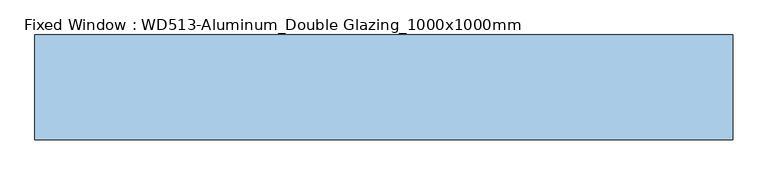
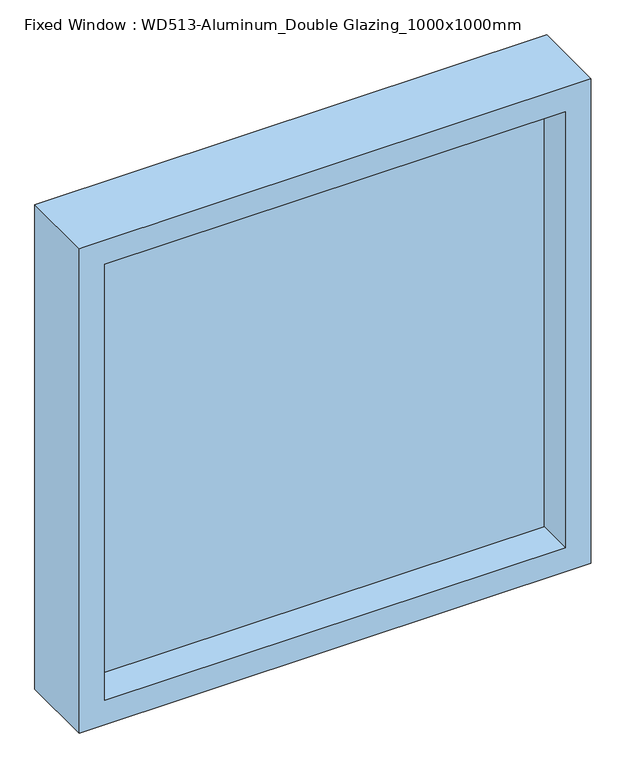
"""IFC4 building model written with IfcOpenShell, lengths in millimetres: window geometry, Fixed Window : WD513-Aluminum_Double Glazing_1000x1000mm."""

import ifcopenshell
import ifcopenshell.guid

model = None  # the IFC model being written
_history = None  # IfcOwnerHistory: only IFC2X3 demands one
_inside = {}  # id of a spatial element -> (the spatial element, [elements in it])
_under = {}  # id of a project, library or spatial element -> (it, [spatial elements below it])
_declared = {}  # id of a project -> (the project, [libraries it declares])
_typed = {}  # id of a type object -> (the type object, [elements of that type])
_made_of = {}  # id of a material, layer set ... -> (it, [elements and type objects made of it])


def new_model(schema):
    """Start an empty IFC model of exactly this schema.

    Asked for "IFC4X3", IfcOpenShell would pick the latest addendum, in which some entities
    have other attributes; the version numbers below select the first issue.
    IFC2X3 requires an IfcOwnerHistory on every rooted entity: one is made here for all.
    """
    global model, _history
    if schema == "IFC4X3":
        model = ifcopenshell.file(schema_version=(4, 3, 0, 0))
    else:
        model = ifcopenshell.file(schema=schema)
    _inside.clear()
    _under.clear()
    _declared.clear()
    _typed.clear()
    _made_of.clear()
    _history = None
    if model.schema == "IFC2X3":
        org = make("IfcOrganization", Name="unknown")
        user = make(
            "IfcPersonAndOrganization",
            ThePerson=make("IfcPerson", FamilyName="unknown"),
            TheOrganization=org,
        )
        app = make(
            "IfcApplication",
            ApplicationDeveloper=org,
            Version="unknown",
            ApplicationFullName="unknown",
            ApplicationIdentifier="unknown",
        )
        _history = make(
            "IfcOwnerHistory",
            OwningUser=user,
            OwningApplication=app,
            ChangeAction="ADDED",
            CreationDate=0,
        )
    return model


def make(cls, **values):
    """One entity of the class cls with the attributes given. An attribute that is None is left unset."""
    return model.create_entity(
        cls, **{name: value for name, value in values.items() if value is not None}
    )


def rooted(cls, **values):
    """An entity with a GlobalId (a new one), such as an element, a storey or a relation."""
    return make(cls, GlobalId=ifcopenshell.guid.new(), OwnerHistory=_history, **values)


def si_unit(unit_type, name, prefix=None):
    """IfcSIUnit, for example si_unit("LENGTHUNIT", "METRE", prefix="MILLI")."""
    return make("IfcSIUnit", UnitType=unit_type, Prefix=prefix, Name=name)


def assignment(units):
    """IfcUnitAssignment: the units of a project."""
    return None if units is None else make("IfcUnitAssignment", Units=units)


def point(xyz):
    """IfcCartesianPoint."""
    return None if xyz is None else make("IfcCartesianPoint", Coordinates=xyz)


def direction(xyz):
    """IfcDirection."""
    return None if xyz is None else make("IfcDirection", DirectionRatios=xyz)


def frame(location, z_axis=None, x_axis=None):
    """IfcAxis2Placement3D, a coordinate frame: its origin and axes. An axis left out is left unset."""
    return make(
        "IfcAxis2Placement3D",
        Location=point(location),
        Axis=direction(z_axis),
        RefDirection=direction(x_axis),
    )


def origin():
    """The frame at (0, 0, 0) with its axes left unset."""
    return frame((0.0, 0.0, 0.0))


def place(relative_to, where):
    """IfcLocalPlacement: puts the frame where relative to a parent placement (None: the world)."""
    return make(
        "IfcLocalPlacement", PlacementRelTo=relative_to, RelativePlacement=where
    )


def context(
    kind, dimensions, precision=None, world=None, true_north=None, identifier=None
):
    """IfcGeometricRepresentationContext, for example the 3D "Model" context."""
    return make(
        "IfcGeometricRepresentationContext",
        ContextIdentifier=identifier,
        ContextType=kind,
        CoordinateSpaceDimension=dimensions,
        Precision=precision,
        WorldCoordinateSystem=world,
        TrueNorth=true_north,
    )


def project(units=None, contexts=None):
    """IfcProject with its units and contexts."""
    return rooted(
        "IfcProject",
        Name="project",
        RepresentationContexts=contexts,
        UnitsInContext=assignment(units),
    )


def spatial(cls, under=None, at=None, **own):
    """A site, building, storey or space (cls), placed at a placement, below another one or the project."""
    s = rooted(cls, ObjectPlacement=at, **own)
    if under is not None:
        _under.setdefault(under.id(), (under, []))[1].append(s)
    return s


def polyline(points):
    """IfcPolyline through the points."""
    return make("IfcPolyline", Points=[point(p) for p in points])


def outline(outer, holes=None, kind="AREA"):
    """IfcArbitraryClosedProfileDef: a profile drawn as a closed curve; with holes, ...WithVoids."""
    if holes is None:
        return make("IfcArbitraryClosedProfileDef", ProfileType=kind, OuterCurve=outer)
    return make(
        "IfcArbitraryProfileDefWithVoids",
        ProfileType=kind,
        OuterCurve=outer,
        InnerCurves=holes,
    )


def extrude(swept, where, along, depth):
    """IfcExtrudedAreaSolid: the profile swept, set in the frame where, extruded along a direction by depth."""
    return make(
        "IfcExtrudedAreaSolid",
        SweptArea=swept,
        Position=where,
        ExtrudedDirection=direction(along),
        Depth=depth,
    )


def shape(context_of_items, identifier, shape_type, items):
    """IfcShapeRepresentation: the items that make up one representation, for example the "Body"."""
    return make(
        "IfcShapeRepresentation",
        ContextOfItems=context_of_items,
        RepresentationIdentifier=identifier,
        RepresentationType=shape_type,
        Items=items,
    )


def source(mapping_origin, context_of_items, identifier, shape_type, items):
    """IfcRepresentationMap: a shape defined once, which mapped items show again and again."""
    return make(
        "IfcRepresentationMap",
        MappingOrigin=mapping_origin,
        MappedRepresentation=shape(context_of_items, identifier, shape_type, items),
    )


def transform(
    local_origin,
    x_axis=None,
    y_axis=None,
    z_axis=None,
    scale=None,
    scale2=None,
    scale3=None,
    uniform=True,
):
    """IfcCartesianTransformationOperator3D, or its non-uniform kind. x_axis, y_axis, z_axis: its Axis1, 2, 3."""
    if uniform:
        return make(
            "IfcCartesianTransformationOperator3D",
            Axis1=direction(x_axis),
            Axis2=direction(y_axis),
            LocalOrigin=point(local_origin),
            Scale=scale,
            Axis3=direction(z_axis),
        )
    return make(
        "IfcCartesianTransformationOperator3DnonUniform",
        Axis1=direction(x_axis),
        Axis2=direction(y_axis),
        LocalOrigin=point(local_origin),
        Scale=scale,
        Axis3=direction(z_axis),
        Scale2=scale2,
        Scale3=scale3,
    )


def mapped(mapping_source, mapping_target):
    """IfcMappedItem: shows the shape of a source again, moved by a transform."""
    return make(
        "IfcMappedItem", MappingSource=mapping_source, MappingTarget=mapping_target
    )


def made_of(thing, what):
    """Note that an element or type object is made of a material, layer set ...; save() writes the relation."""
    if what is not None:
        _made_of.setdefault(what.id(), (what, []))[1].append(thing)
    return thing


def element(
    cls,
    number,
    at=None,
    inside=None,
    cuts=None,
    type_object=None,
    material=None,
    context=None,
    identifier="Body",
    shape_type=None,
    held_by="IfcProductDefinitionShape",
    body=None,
    shapes=None,
    **own,
):
    """One element of the class cls, such as IfcWall. Its Tag is "e" and its number.

    at: its placement. inside: the storey or other place that contains it. cuts: it is an
    opening in that element (IfcRelVoidsElement). A single representation is given by context,
    identifier, shape_type and body (its items); several are given by shapes. held_by: the class
    of the entity that holds the representations. save() writes the other relations.
    """
    e = rooted(cls, Tag="e%d" % number, ObjectPlacement=at, **own)
    if body is not None:
        shapes = [shape(context, identifier, shape_type, body)]
    if shapes is not None:
        e.Representation = make(held_by, Representations=shapes)
    if inside is not None:
        _inside.setdefault(inside.id(), (inside, []))[1].append(e)
    if cuts is not None:
        rooted(
            "IfcRelVoidsElement", RelatingBuildingElement=cuts, RelatedOpeningElement=e
        )
    if type_object is not None:
        _typed.setdefault(type_object.id(), (type_object, []))[1].append(e)
    return made_of(e, material)


def aggregate(whole, parts):
    """IfcRelAggregates: a whole, such as a stair, and the parts it consists of."""
    return rooted("IfcRelAggregates", RelatingObject=whole, RelatedObjects=parts)


def save(model, path):
    """Write the relations noted so far, then the file.

    IfcRelAggregates (storeys below a building ...), IfcRelContainedInSpatialStructure (elements
    in a storey), IfcRelDefinesByType, IfcRelAssociatesMaterial and IfcRelDeclares: one each for
    every whole, place, type object, material and project.
    """
    for whole, parts in _under.values():
        aggregate(whole, parts)
    for where, things in _inside.values():
        rooted(
            "IfcRelContainedInSpatialStructure",
            RelatedElements=things,
            RelatingStructure=where,
        )
    for kind, things in _typed.values():
        rooted("IfcRelDefinesByType", RelatedObjects=things, RelatingType=kind)
    for what, things in _made_of.values():
        rooted("IfcRelAssociatesMaterial", RelatedObjects=things, RelatingMaterial=what)
    for by, libraries in _declared.values():
        rooted("IfcRelDeclares", RelatingContext=by, RelatedDefinitions=libraries)
    model.write(path)


def fixed_window_wd513_aluminum_double_glazing_1000x1000mm_e073f05b(model_context):
    return source(origin(), model_context, "Body", "SweptSolid", [
        extrude(outline(polyline([(-450.0, 3.0), (450.0, 3.0), (450.0, -3.0), (-450.0, -3.0), (-450.0, 3.0)])), frame((0.0, 0.0, 850.0), z_axis=(0.0, 0.0, 1.0), x_axis=(1.0, 0.0, 0.0)), (0.0, 0.0, 1.0), 900.0),
        extrude(outline(polyline([(1800.0, -500.0), (800.0, -500.0), (800.0, 500.0), (1800.0, 500.0), (1800.0, -500.0)]), holes=[polyline([(1750.0, -450.0), (1750.0, 450.0), (850.0, 450.0), (850.0, -450.0), (1750.0, -450.0)])]), frame((0.0, -75.0, 0.0), z_axis=(0.0, 1.0, 0.0), x_axis=(0.0, 0.0, 1.0)), (0.0, 0.0, 1.0), 150.0),
    ])


if __name__ == "__main__":
    model = new_model("IFC4")
    model_context = context("Model", 3, world=origin())
    ifc_project = project(units=[si_unit("LENGTHUNIT", "METRE", prefix="MILLI")], contexts=[model_context])
    site = spatial("IfcSite", under=ifc_project)
    building = spatial("IfcBuilding", under=site)
    placement = place(None, origin())
    fixed_window_wd513_aluminum_double_glazing_1000x1000mm_shape = fixed_window_wd513_aluminum_double_glazing_1000x1000mm_e073f05b(model_context)
    element("IfcWindow", 1, ObjectType="Fixed Window : WD513-Aluminum_Double Glazing_1000x1000mm", at=placement, inside=building, context=model_context, shape_type="MappedRepresentation", body=[
        mapped(fixed_window_wd513_aluminum_double_glazing_1000x1000mm_shape, transform((0.0, 0.0, 0.0), x_axis=(1.0, 0.0, 0.0), y_axis=(0.0, 1.0, 0.0), z_axis=(0.0, 0.0, 1.0))),
    ])
    save(model, "model.ifc")

# Revit data of these elements
# Type "Fixed Window : WD513-Aluminum_Double Glazing_1000x1000mm"
#   Type Mark = "193"
#   Analytic Construction = "<None>"
#   창 두께 = 150 mm
#   Height = 1000 mm
#   절반 창 두께 = 75 mm
#   기본 씰 높이 = 800 mm
#   Width = 1000 mm
#   Define Thermal Properties by = 1
#   창 패널 = AW2 창 패널
#   창 프레임 = A04AQ127-00002_Aluminum Window_None FP
#   Wall Closure = (empty or 0)
# Element 1 (IfcWindow, "Fixed Window : WD513-Aluminum_Double Glazing_1000x1000mm")
#   Materials on its faces: "A04AQ127-00002_Aluminum Window_None FP", "AW2 창 패널"
# Materials
#   "AW2 창 패널": class "유리", colour RGB 0 0 255, transparency 0.75
#   "A04AQ127-00002_Aluminum Window_None FP": class "금속", colour RGB 247 247 247, transparency 0, W00) Work Master Code = "A04AQ127-00002", W01) Work Master_Lv1 = "Finishing Work", W02) Work Master_Lv2 = "Door & Window Work", W03) Work Master_Spec.1 = "Aluminum Window", W04) Work Master_Spec.2 = "Fire Protective Rating: N/A", W05) Work Master_Spec.3 = "w/ Hardware & Accessories", Cost = 0
